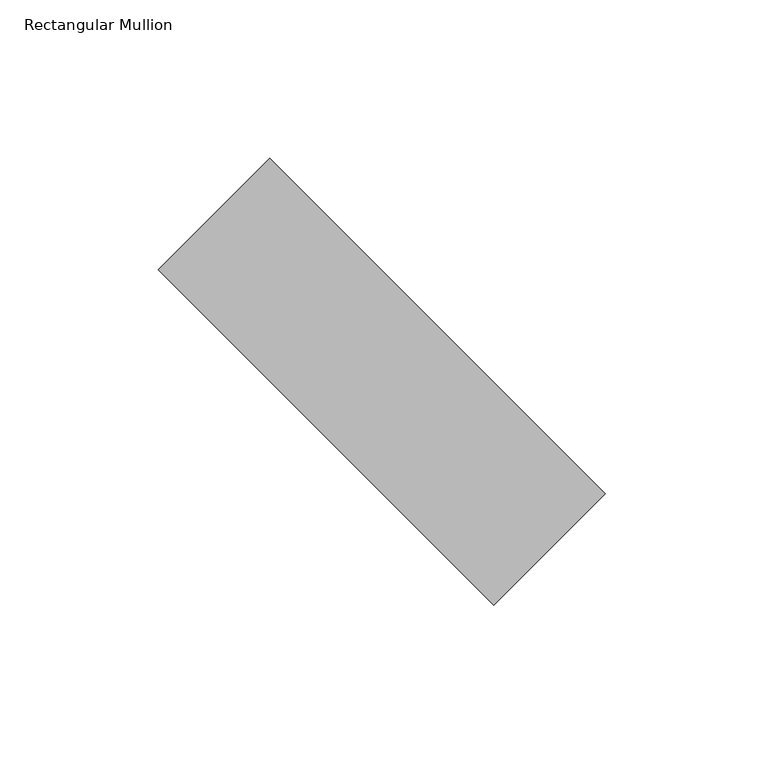
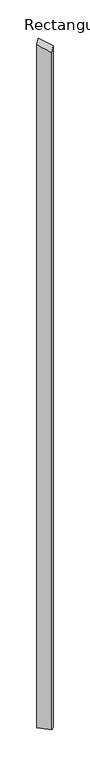
"""IFC4 building model written with IfcOpenShell, lengths in millimetres: member geometry, Rectangular Mullion : tilted mullions."""

from ifc_helpers import new_model, si_unit, origin, place, context, project, spatial, faceted_brep, source, transform, mapped, element, save


def rectangular_mullion_749d1d03(model_context):
    return source(origin(), model_context, "Body", "Brep", [
        faceted_brep([(-35.3553391, 70.7106781, -7999.1607688), (70.7106781, -35.3553391, -7999.1607688), (35.3553391, -70.7106781, -7999.1607688), (-70.7106781, 35.3553391, -7999.1607688), (-70.7106781, 35.3553391, 10.0516542), (-35.3553391, 70.7106781, 55.0905224), (35.3553391, -70.7106781, -55.0905224), (70.7106781, -35.3553391, -10.0516542)], [[[0, 1, 2, 3]], [[4, 5, 0, 3]], [[6, 4, 3, 2]], [[7, 6, 2, 1]], [[5, 7, 1, 0]], [[5, 4, 6, 7]]]),
    ])


if __name__ == "__main__":
    model = new_model("IFC4")
    model_context = context("Model", 3, world=origin())
    ifc_project = project(units=[si_unit("LENGTHUNIT", "METRE", prefix="MILLI")], contexts=[model_context])
    site = spatial("IfcSite", under=ifc_project)
    building = spatial("IfcBuilding", under=site)
    placement = place(None, origin())
    rectangular_mullion_shape = rectangular_mullion_749d1d03(model_context)
    element("IfcMember", 1, ObjectType="Rectangular Mullion : tilted mullions", at=placement, inside=building, context=model_context, shape_type="MappedRepresentation", body=[
        mapped(rectangular_mullion_shape, transform((0.0, 0.0, 0.0), x_axis=(1.0, 0.0, 0.0), y_axis=(0.0, 1.0, 0.0), z_axis=(0.0, 0.0, 1.0))),
    ])
    save(model, "model.ifc")

# Revit data of these elements
# Type "Rectangular Mullion : tilted mullions"
#   built-in parameter 1007304 = 0.492126 (stored number, unit not read)
#   built-in parameter 1007301 = 0.082021 (stored number, unit not read)
#   built-in parameter 1007300 = 0.082021 (stored number, unit not read)
# Element 1 (IfcMember, "Rectangular Mullion : tilted mullions")
#   Materials on its faces: "Aluminum"
# Materials
#   "Aluminum": class "Metal", colour RGB 244 244 244, transparency 0, Description = "Aluminum 6061", Cost = 0
